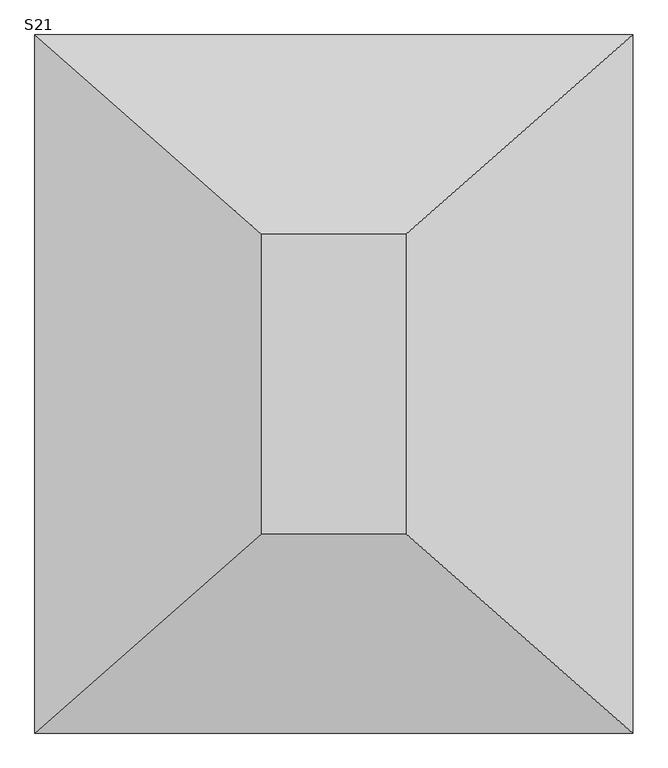
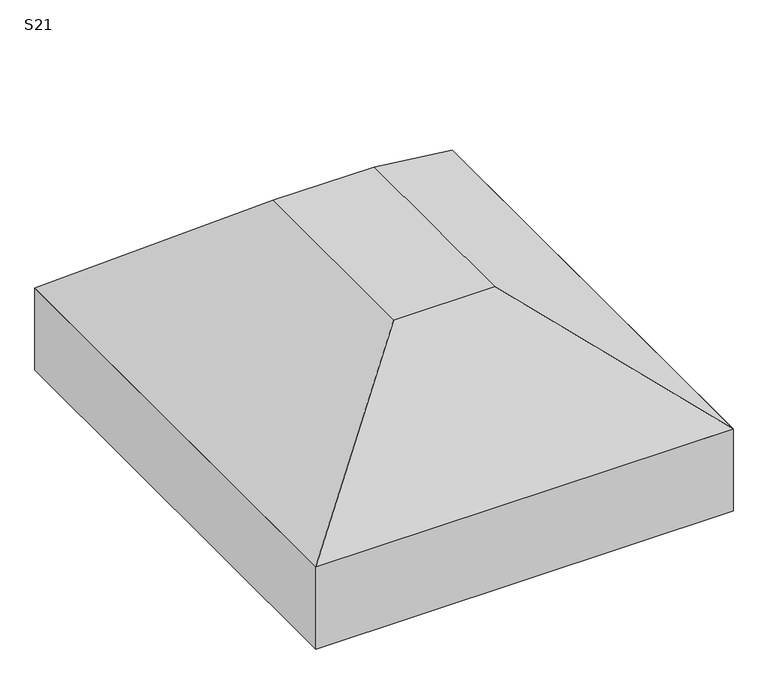
"""IFC4 building model written with IfcOpenShell, lengths in millimetres: fastener geometry, TQS - Sapata : S21."""

import ifcopenshell
import ifcopenshell.guid

model = None  # the IFC model being written
_history = None  # IfcOwnerHistory: only IFC2X3 demands one
_inside = {}  # id of a spatial element -> (the spatial element, [elements in it])
_under = {}  # id of a project, library or spatial element -> (it, [spatial elements below it])
_declared = {}  # id of a project -> (the project, [libraries it declares])
_typed = {}  # id of a type object -> (the type object, [elements of that type])
_made_of = {}  # id of a material, layer set ... -> (it, [elements and type objects made of it])


def new_model(schema):
    """Start an empty IFC model of exactly this schema.

    Asked for "IFC4X3", IfcOpenShell would pick the latest addendum, in which some entities
    have other attributes; the version numbers below select the first issue.
    IFC2X3 requires an IfcOwnerHistory on every rooted entity: one is made here for all.
    """
    global model, _history
    if schema == "IFC4X3":
        model = ifcopenshell.file(schema_version=(4, 3, 0, 0))
    else:
        model = ifcopenshell.file(schema=schema)
    _inside.clear()
    _under.clear()
    _declared.clear()
    _typed.clear()
    _made_of.clear()
    _history = None
    if model.schema == "IFC2X3":
        org = make("IfcOrganization", Name="unknown")
        user = make(
            "IfcPersonAndOrganization",
            ThePerson=make("IfcPerson", FamilyName="unknown"),
            TheOrganization=org,
        )
        app = make(
            "IfcApplication",
            ApplicationDeveloper=org,
            Version="unknown",
            ApplicationFullName="unknown",
            ApplicationIdentifier="unknown",
        )
        _history = make(
            "IfcOwnerHistory",
            OwningUser=user,
            OwningApplication=app,
            ChangeAction="ADDED",
            CreationDate=0,
        )
    return model


def make(cls, **values):
    """One entity of the class cls with the attributes given. An attribute that is None is left unset."""
    return model.create_entity(
        cls, **{name: value for name, value in values.items() if value is not None}
    )


def rooted(cls, **values):
    """An entity with a GlobalId (a new one), such as an element, a storey or a relation."""
    return make(cls, GlobalId=ifcopenshell.guid.new(), OwnerHistory=_history, **values)


def si_unit(unit_type, name, prefix=None):
    """IfcSIUnit, for example si_unit("LENGTHUNIT", "METRE", prefix="MILLI")."""
    return make("IfcSIUnit", UnitType=unit_type, Prefix=prefix, Name=name)


def assignment(units):
    """IfcUnitAssignment: the units of a project."""
    return None if units is None else make("IfcUnitAssignment", Units=units)


def point(xyz):
    """IfcCartesianPoint."""
    return None if xyz is None else make("IfcCartesianPoint", Coordinates=xyz)


def direction(xyz):
    """IfcDirection."""
    return None if xyz is None else make("IfcDirection", DirectionRatios=xyz)


def frame(location, z_axis=None, x_axis=None):
    """IfcAxis2Placement3D, a coordinate frame: its origin and axes. An axis left out is left unset."""
    return make(
        "IfcAxis2Placement3D",
        Location=point(location),
        Axis=direction(z_axis),
        RefDirection=direction(x_axis),
    )


def origin():
    """The frame at (0, 0, 0) with its axes left unset."""
    return frame((0.0, 0.0, 0.0))


def place(relative_to, where):
    """IfcLocalPlacement: puts the frame where relative to a parent placement (None: the world)."""
    return make(
        "IfcLocalPlacement", PlacementRelTo=relative_to, RelativePlacement=where
    )


def context(
    kind, dimensions, precision=None, world=None, true_north=None, identifier=None
):
    """IfcGeometricRepresentationContext, for example the 3D "Model" context."""
    return make(
        "IfcGeometricRepresentationContext",
        ContextIdentifier=identifier,
        ContextType=kind,
        CoordinateSpaceDimension=dimensions,
        Precision=precision,
        WorldCoordinateSystem=world,
        TrueNorth=true_north,
    )


def project(units=None, contexts=None):
    """IfcProject with its units and contexts."""
    return rooted(
        "IfcProject",
        Name="project",
        RepresentationContexts=contexts,
        UnitsInContext=assignment(units),
    )


def spatial(cls, under=None, at=None, **own):
    """A site, building, storey or space (cls), placed at a placement, below another one or the project."""
    s = rooted(cls, ObjectPlacement=at, **own)
    if under is not None:
        _under.setdefault(under.id(), (under, []))[1].append(s)
    return s


def polyline(points):
    """IfcPolyline through the points."""
    return make("IfcPolyline", Points=[point(p) for p in points])


def outline(outer, holes=None, kind="AREA"):
    """IfcArbitraryClosedProfileDef: a profile drawn as a closed curve; with holes, ...WithVoids."""
    if holes is None:
        return make("IfcArbitraryClosedProfileDef", ProfileType=kind, OuterCurve=outer)
    return make(
        "IfcArbitraryProfileDefWithVoids",
        ProfileType=kind,
        OuterCurve=outer,
        InnerCurves=holes,
    )


def extrude(swept, where, along, depth):
    """IfcExtrudedAreaSolid: the profile swept, set in the frame where, extruded along a direction by depth."""
    return make(
        "IfcExtrudedAreaSolid",
        SweptArea=swept,
        Position=where,
        ExtrudedDirection=direction(along),
        Depth=depth,
    )


def faces_of(points, faces, orient=None, outer=None):
    """IfcFace entities. A face is a list of loops; a loop is a list of indices into points, from 0.

    orient and outer hold one flag for each loop. By default every Orientation is true, the
    first loop of a face is its IfcFaceOuterBound and the others are IfcFaceBound.
    """
    made = []
    for i, loops in enumerate(faces):
        bounds = []
        for j, loop in enumerate(loops):
            is_outer = j == 0 if outer is None else outer[i][j]
            bounds.append(
                make(
                    "IfcFaceOuterBound" if is_outer else "IfcFaceBound",
                    Bound=make("IfcPolyLoop", Polygon=[points[k] for k in loop]),
                    Orientation=True if orient is None else orient[i][j],
                )
            )
        made.append(make("IfcFace", Bounds=bounds))
    return made


def faceted_brep(points, faces, orient=None, outer=None, voids=None):
    """IfcFacetedBrep: a solid bounded by flat faces; with voids (closed shells), ...WithVoids."""
    shared = [point(p) for p in points]
    hull = make("IfcClosedShell", CfsFaces=faces_of(shared, faces, orient, outer))
    if voids is None:
        return make("IfcFacetedBrep", Outer=hull)
    return make(
        "IfcFacetedBrepWithVoids",
        Outer=hull,
        Voids=[
            make(cls, CfsFaces=faces_of(shared, fs, o, b)) for cls, fs, o, b in voids
        ],
    )


def shape(context_of_items, identifier, shape_type, items):
    """IfcShapeRepresentation: the items that make up one representation, for example the "Body"."""
    return make(
        "IfcShapeRepresentation",
        ContextOfItems=context_of_items,
        RepresentationIdentifier=identifier,
        RepresentationType=shape_type,
        Items=items,
    )


def source(mapping_origin, context_of_items, identifier, shape_type, items):
    """IfcRepresentationMap: a shape defined once, which mapped items show again and again."""
    return make(
        "IfcRepresentationMap",
        MappingOrigin=mapping_origin,
        MappedRepresentation=shape(context_of_items, identifier, shape_type, items),
    )


def transform(
    local_origin,
    x_axis=None,
    y_axis=None,
    z_axis=None,
    scale=None,
    scale2=None,
    scale3=None,
    uniform=True,
):
    """IfcCartesianTransformationOperator3D, or its non-uniform kind. x_axis, y_axis, z_axis: its Axis1, 2, 3."""
    if uniform:
        return make(
            "IfcCartesianTransformationOperator3D",
            Axis1=direction(x_axis),
            Axis2=direction(y_axis),
            LocalOrigin=point(local_origin),
            Scale=scale,
            Axis3=direction(z_axis),
        )
    return make(
        "IfcCartesianTransformationOperator3DnonUniform",
        Axis1=direction(x_axis),
        Axis2=direction(y_axis),
        LocalOrigin=point(local_origin),
        Scale=scale,
        Axis3=direction(z_axis),
        Scale2=scale2,
        Scale3=scale3,
    )


def mapped(mapping_source, mapping_target):
    """IfcMappedItem: shows the shape of a source again, moved by a transform."""
    return make(
        "IfcMappedItem", MappingSource=mapping_source, MappingTarget=mapping_target
    )


def made_of(thing, what):
    """Note that an element or type object is made of a material, layer set ...; save() writes the relation."""
    if what is not None:
        _made_of.setdefault(what.id(), (what, []))[1].append(thing)
    return thing


def element(
    cls,
    number,
    at=None,
    inside=None,
    cuts=None,
    type_object=None,
    material=None,
    context=None,
    identifier="Body",
    shape_type=None,
    held_by="IfcProductDefinitionShape",
    body=None,
    shapes=None,
    **own,
):
    """One element of the class cls, such as IfcWall. Its Tag is "e" and its number.

    at: its placement. inside: the storey or other place that contains it. cuts: it is an
    opening in that element (IfcRelVoidsElement). A single representation is given by context,
    identifier, shape_type and body (its items); several are given by shapes. held_by: the class
    of the entity that holds the representations. save() writes the other relations.
    """
    e = rooted(cls, Tag="e%d" % number, ObjectPlacement=at, **own)
    if body is not None:
        shapes = [shape(context, identifier, shape_type, body)]
    if shapes is not None:
        e.Representation = make(held_by, Representations=shapes)
    if inside is not None:
        _inside.setdefault(inside.id(), (inside, []))[1].append(e)
    if cuts is not None:
        rooted(
            "IfcRelVoidsElement", RelatingBuildingElement=cuts, RelatedOpeningElement=e
        )
    if type_object is not None:
        _typed.setdefault(type_object.id(), (type_object, []))[1].append(e)
    return made_of(e, material)


def aggregate(whole, parts):
    """IfcRelAggregates: a whole, such as a stair, and the parts it consists of."""
    return rooted("IfcRelAggregates", RelatingObject=whole, RelatedObjects=parts)


def save(model, path):
    """Write the relations noted so far, then the file.

    IfcRelAggregates (storeys below a building ...), IfcRelContainedInSpatialStructure (elements
    in a storey), IfcRelDefinesByType, IfcRelAssociatesMaterial and IfcRelDeclares: one each for
    every whole, place, type object, material and project.
    """
    for whole, parts in _under.values():
        aggregate(whole, parts)
    for where, things in _inside.values():
        rooted(
            "IfcRelContainedInSpatialStructure",
            RelatedElements=things,
            RelatingStructure=where,
        )
    for kind, things in _typed.values():
        rooted("IfcRelDefinesByType", RelatedObjects=things, RelatingType=kind)
    for what, things in _made_of.values():
        rooted("IfcRelAssociatesMaterial", RelatedObjects=things, RelatingMaterial=what)
    for by, libraries in _declared.values():
        rooted("IfcRelDeclares", RelatingContext=by, RelatedDefinitions=libraries)
    model.write(path)


def s21_dbbb6426(model_context):
    return source(origin(), model_context, "Body", "SolidModel", [
        faceted_brep([(-55.0, 100.0, 0.0), (-345.0, 100.0, 0.0), (-345.0, -500.0, 0.0), (-55.0, -500.0, 0.0), (400.0, 500.0, -350.0), (400.0, -900.0, -350.0), (-800.0, -900.0, -350.0), (-800.0, 500.0, -350.0)], [[[0, 1, 2, 3]], [[4, 5, 6, 7]], [[4, 7, 1, 0]], [[7, 6, 2, 1]], [[6, 5, 3, 2]], [[5, 4, 0, 3]]]),
        extrude(outline(polyline([(400.0, 500.0), (400.0, -900.0), (-800.0, -900.0), (-800.0, 500.0), (400.0, 500.0)])), frame((0.0, 0.0, -600.0), z_axis=(0.0, 0.0, 1.0), x_axis=(1.0, 0.0, 0.0)), (0.0, 0.0, 1.0), 250.0),
    ])


if __name__ == "__main__":
    model = new_model("IFC4")
    model_context = context("Model", 3, world=origin())
    ifc_project = project(units=[si_unit("LENGTHUNIT", "METRE", prefix="MILLI")], contexts=[model_context])
    site = spatial("IfcSite", under=ifc_project)
    building = spatial("IfcBuilding", under=site)
    placement = place(None, origin())
    s21_shape = s21_dbbb6426(model_context)
    element("IfcFastener", 1, ObjectType="TQS - Sapata : S21", at=placement, inside=building, context=model_context, shape_type="MappedRepresentation", body=[
        mapped(s21_shape, transform((0.0, 0.0, 0.0), x_axis=(1.0, 0.0, 0.0), y_axis=(0.0, 1.0, 0.0), z_axis=(0.0, 0.0, 1.0))),
    ])
    save(model, "model.ifc")

# Revit data of these elements
# Type "TQS - Sapata : S21"
#   TY = 0.60 m
#   TX = 0.29 m
#   HS = 0.60 m
#   H0 = 0.25 m
#   EXCYABS = 0.70 m
#   EXCY = 0.00 m
#   EXCXABS = 0.60 m
#   EXCX = 0.00 m
#   DIMY = 1.40 m
#   DIMX = 1.20 m
#   Material estrutural = Concreto - Concreto concretado no local
#   Width = 0
#   Length = 0
# Element 1 (IfcFastener, "TQS - Sapata : S21")
#   Materials on its faces: "Concreto - Concreto concretado no local"
# Materials
#   "Concreto - Concreto concretado no local": class "Concreto", colour RGB 192 192 192, transparency 0
